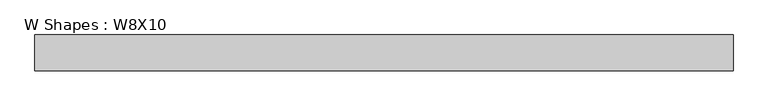
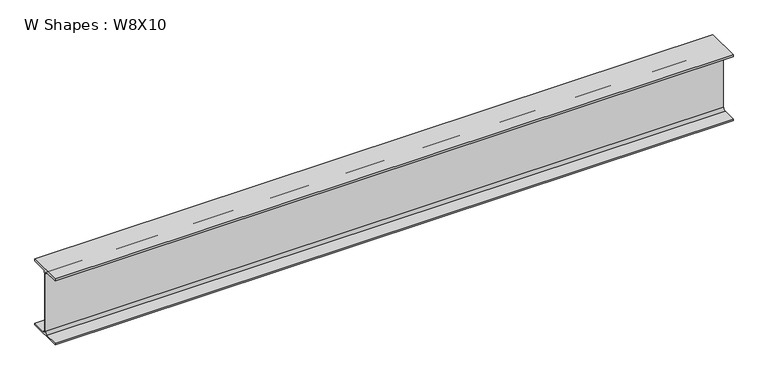
"""IFC4 building model written with IfcOpenShell, lengths in millimetres: beam geometry, W Shapes : W8X10."""

from ifc_helpers import new_model, si_unit, point, frame, frame_2d, origin, place, context, project, spatial, polyline, circle_curve, trimmed, segment, composite_curve, outline, extrude, source, transform, mapped, element, save


def w_shapes_w8x10_a5119e61(model_context):
    return source(origin(), model_context, "Body", "SweptSolid", [
        extrude(outline(composite_curve([segment(polyline([(50.038, -94.996), (50.038, -100.203), (-50.038, -100.203), (-50.038, -94.996), (-9.779, -94.996)]), True, "CONTINUOUS"), segment(trimmed(circle_curve(frame_2d((-9.779, -87.376)), 7.62), [point((-9.779, -94.996))], [point((-2.159, -87.376))], True, "CARTESIAN"), True, "CONTINUOUS"), segment(polyline([(-2.159, -87.376), (-2.159, 87.376)]), True, "CONTINUOUS"), segment(trimmed(circle_curve(frame_2d((-9.779, 87.376)), 7.62), [point((-2.159, 87.376))], [point((-9.779, 94.996))], True, "CARTESIAN"), True, "CONTINUOUS"), segment(polyline([(-9.779, 94.996), (-50.038, 94.996), (-50.038, 100.203), (50.038, 100.203), (50.038, 94.996), (9.779, 94.996)]), True, "CONTINUOUS"), segment(trimmed(circle_curve(frame_2d((9.779, 87.376)), 7.62), [point((9.779, 94.996))], [point((2.159, 87.376))], True, "CARTESIAN"), True, "CONTINUOUS"), segment(polyline([(2.159, 87.376), (2.159, -87.376)]), True, "CONTINUOUS"), segment(trimmed(circle_curve(frame_2d((9.779, -87.376)), 7.62), [point((2.159, -87.376))], [point((9.779, -94.996))], True, "CARTESIAN"), True, "CONTINUOUS"), segment(polyline([(9.779, -94.996), (50.038, -94.996)]), True, "CONTINUOUS")], self_intersect=False)), frame((-974.344, 0.0, 0.0), z_axis=(1.0, 0.0, 0.0), x_axis=(0.0, 1.0, 0.0)), (0.0, 0.0, 1.0), 1948.688),
    ])


if __name__ == "__main__":
    model = new_model("IFC4")
    model_context = context("Model", 3, world=origin())
    ifc_project = project(units=[si_unit("LENGTHUNIT", "METRE", prefix="MILLI")], contexts=[model_context])
    site = spatial("IfcSite", under=ifc_project)
    building = spatial("IfcBuilding", under=site)
    placement = place(None, origin())
    w_shapes_w8x10_shape = w_shapes_w8x10_a5119e61(model_context)
    element("IfcBeam", 1, ObjectType="W Shapes : W8X10", at=placement, inside=building, context=model_context, shape_type="MappedRepresentation", body=[
        mapped(w_shapes_w8x10_shape, transform((0.0, 0.0, 0.0), x_axis=(1.0, 0.0, 0.0), y_axis=(0.0, 1.0, 0.0), z_axis=(0.0, 0.0, 1.0))),
    ])
    save(model, "model.ifc")

# Revit data of these elements
# Type "W Shapes : W8X10"
#   Section Name Key = "W8x10"
#   Assembly Code = "B10"
#   Width = 3.940"
#   Web Thickness = 0.170"
#   Web Fillet = 0.300"
#   Warping Constant = 30.90 in⁶
#   Torsional Moment of Inertia = 0.0426 in⁴
#   Section Area = 2.96 in²
#   Plastic Modulus weak axis = 1.66 in³
#   Plastic Modulus strong axis = 8.87 in³
#   Perimeter = 30.70 ft²/ft
#   Nominal Weight = 10.00 lbf/ft
#   Moment of Inertia weak axis = 2.09 in⁴
#   Moment of Inertia strong axis = 30.80 in⁴
#   Height = 7.890"
#   Flange Thickness = 0.205"
#   Elastic Modulus weak axis = 1.06 in³
#   Elastic Modulus strong axis = 7.81 in³
#   Centroid Vertical = 3.945"
#   Centroid Horizontal = 1.970"
#   Bolt Spacing = 0' - 2 1/4"
#   Length [instance default] = 5' - 0"
#   Structural Material [instance default] = Steel ASTM A992
#   Principal Axes Angle = 0
# Element 1 (IfcBeam, "W Shapes : W8X10")
#   Materials on its faces: "Steel ASTM A992"
# Materials
#   "Steel ASTM A992": class "Metal", colour RGB 199 199 199, transparency 0, Description = "Structural steel 50ksi", Cost = 0
